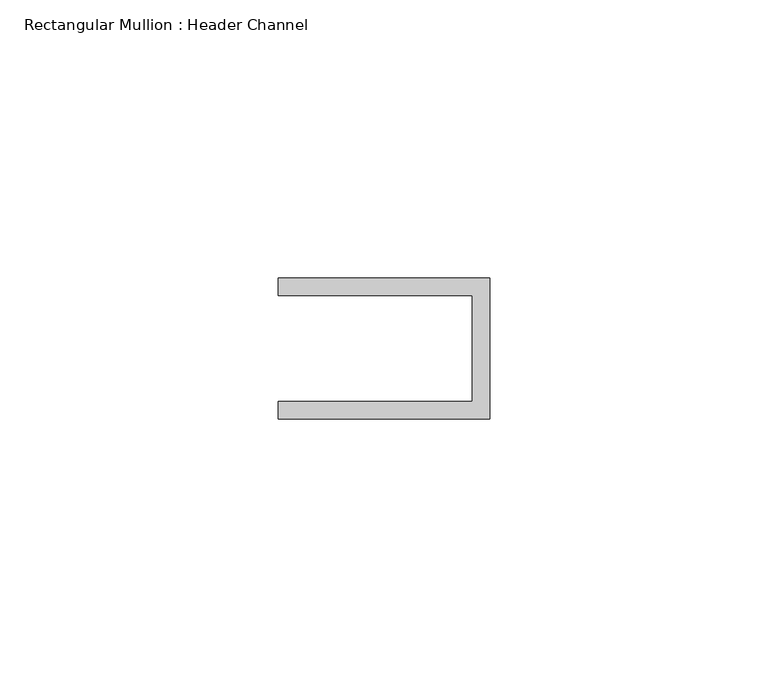
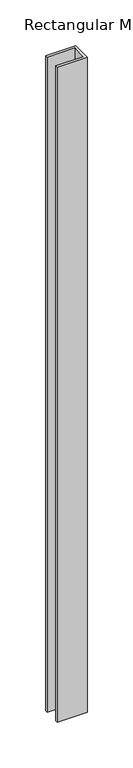
"""IFC4 building model written with IfcOpenShell, lengths in millimetres: member geometry, Rectangular Mullion : Header Channel."""

from ifc_helpers import new_model, si_unit, frame, origin, place, context, project, spatial, polyline, outline, extrude, source, transform, mapped, element, save


def rectangular_mullion_header_channel_b7be825e(model_context):
    return source(origin(), model_context, "Body", "SweptSolid", [
        extrude(outline(polyline([(0.0, 12.7), (0.0, -12.7), (-38.1, -12.7), (-38.1, -9.525), (-3.175, -9.525), (-3.175, 9.525), (-38.1, 9.525), (-38.1, 12.7), (0.0, 12.7)])), frame((0.0, 0.0, -876.6175002), z_axis=(0.0, 0.0, 1.0), x_axis=(1.0, 0.0, 0.0)), (0.0, 0.0, 1.0), 876.6175002),
    ])


if __name__ == "__main__":
    model = new_model("IFC4")
    model_context = context("Model", 3, world=origin())
    ifc_project = project(units=[si_unit("LENGTHUNIT", "METRE", prefix="MILLI")], contexts=[model_context])
    site = spatial("IfcSite", under=ifc_project)
    building = spatial("IfcBuilding", under=site)
    placement = place(None, origin())
    rectangular_mullion_header_channel_shape = rectangular_mullion_header_channel_b7be825e(model_context)
    element("IfcMember", 1, ObjectType="Rectangular Mullion : Header Channel", at=placement, inside=building, context=model_context, shape_type="MappedRepresentation", body=[
        mapped(rectangular_mullion_header_channel_shape, transform((0.0, 0.0, 0.0), x_axis=(1.0, 0.0, 0.0), y_axis=(0.0, 1.0, 0.0), z_axis=(0.0, 0.0, 1.0))),
    ])
    save(model, "model.ifc")

# Revit data of these elements
# Type "Rectangular Mullion : Header Channel"
#   built-in parameter 1007322 = 0.0833333 (stored number, unit not read)
#   built-in parameter 1007321 = -0.03125 (stored number, unit not read)
#   built-in parameter 1007320 = 0.0416667 (stored number, unit not read)
# Element 1 (IfcMember, "Rectangular Mullion : Header Channel")
#   Materials on its faces: "ALUM"
# Materials
#   "ALUM": class "Generic", colour RGB 157 157 157, transparency 0, Cost = 0
